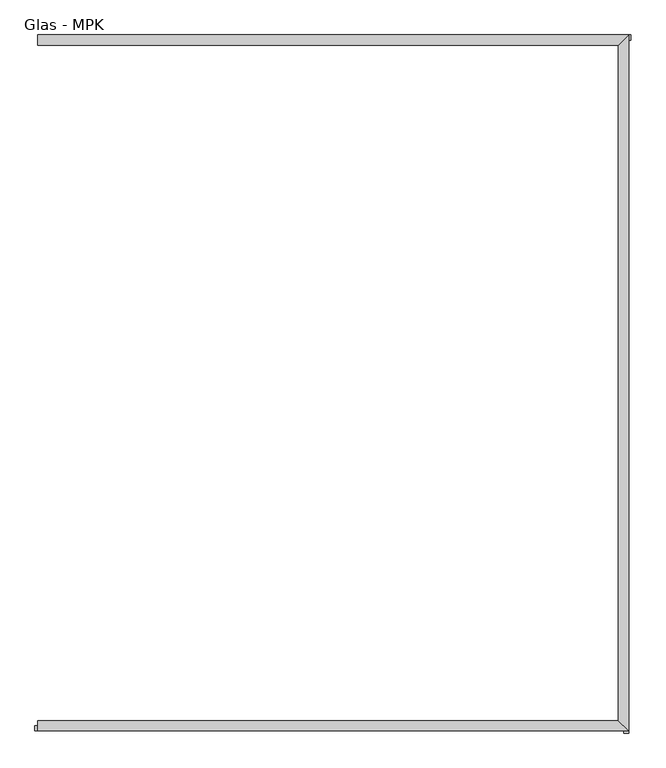
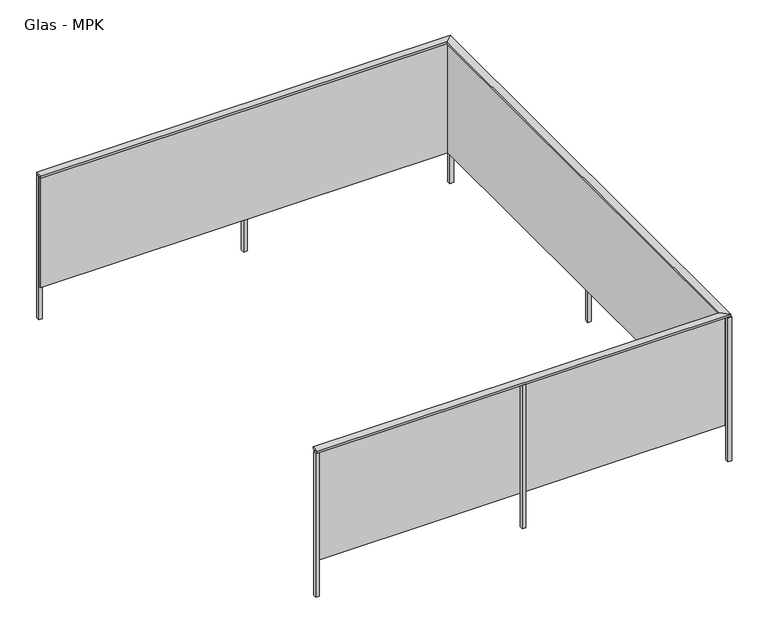
"""IFC4 building model written with IfcOpenShell, lengths in millimetres: railing geometry, Glas - MPK."""

import ifcopenshell
import ifcopenshell.guid

model = None  # the IFC model being written
_history = None  # IfcOwnerHistory: only IFC2X3 demands one
_inside = {}  # id of a spatial element -> (the spatial element, [elements in it])
_under = {}  # id of a project, library or spatial element -> (it, [spatial elements below it])
_declared = {}  # id of a project -> (the project, [libraries it declares])
_typed = {}  # id of a type object -> (the type object, [elements of that type])
_made_of = {}  # id of a material, layer set ... -> (it, [elements and type objects made of it])


def new_model(schema):
    """Start an empty IFC model of exactly this schema.

    Asked for "IFC4X3", IfcOpenShell would pick the latest addendum, in which some entities
    have other attributes; the version numbers below select the first issue.
    IFC2X3 requires an IfcOwnerHistory on every rooted entity: one is made here for all.
    """
    global model, _history
    if schema == "IFC4X3":
        model = ifcopenshell.file(schema_version=(4, 3, 0, 0))
    else:
        model = ifcopenshell.file(schema=schema)
    _inside.clear()
    _under.clear()
    _declared.clear()
    _typed.clear()
    _made_of.clear()
    _history = None
    if model.schema == "IFC2X3":
        org = make("IfcOrganization", Name="unknown")
        user = make(
            "IfcPersonAndOrganization",
            ThePerson=make("IfcPerson", FamilyName="unknown"),
            TheOrganization=org,
        )
        app = make(
            "IfcApplication",
            ApplicationDeveloper=org,
            Version="unknown",
            ApplicationFullName="unknown",
            ApplicationIdentifier="unknown",
        )
        _history = make(
            "IfcOwnerHistory",
            OwningUser=user,
            OwningApplication=app,
            ChangeAction="ADDED",
            CreationDate=0,
        )
    return model


def make(cls, **values):
    """One entity of the class cls with the attributes given. An attribute that is None is left unset."""
    return model.create_entity(
        cls, **{name: value for name, value in values.items() if value is not None}
    )


def rooted(cls, **values):
    """An entity with a GlobalId (a new one), such as an element, a storey or a relation."""
    return make(cls, GlobalId=ifcopenshell.guid.new(), OwnerHistory=_history, **values)


def si_unit(unit_type, name, prefix=None):
    """IfcSIUnit, for example si_unit("LENGTHUNIT", "METRE", prefix="MILLI")."""
    return make("IfcSIUnit", UnitType=unit_type, Prefix=prefix, Name=name)


def assignment(units):
    """IfcUnitAssignment: the units of a project."""
    return None if units is None else make("IfcUnitAssignment", Units=units)


def point(xyz):
    """IfcCartesianPoint."""
    return None if xyz is None else make("IfcCartesianPoint", Coordinates=xyz)


def direction(xyz):
    """IfcDirection."""
    return None if xyz is None else make("IfcDirection", DirectionRatios=xyz)


def frame(location, z_axis=None, x_axis=None):
    """IfcAxis2Placement3D, a coordinate frame: its origin and axes. An axis left out is left unset."""
    return make(
        "IfcAxis2Placement3D",
        Location=point(location),
        Axis=direction(z_axis),
        RefDirection=direction(x_axis),
    )


def origin():
    """The frame at (0, 0, 0) with its axes left unset."""
    return frame((0.0, 0.0, 0.0))


def place(relative_to, where):
    """IfcLocalPlacement: puts the frame where relative to a parent placement (None: the world)."""
    return make(
        "IfcLocalPlacement", PlacementRelTo=relative_to, RelativePlacement=where
    )


def context(
    kind, dimensions, precision=None, world=None, true_north=None, identifier=None
):
    """IfcGeometricRepresentationContext, for example the 3D "Model" context."""
    return make(
        "IfcGeometricRepresentationContext",
        ContextIdentifier=identifier,
        ContextType=kind,
        CoordinateSpaceDimension=dimensions,
        Precision=precision,
        WorldCoordinateSystem=world,
        TrueNorth=true_north,
    )


def project(units=None, contexts=None):
    """IfcProject with its units and contexts."""
    return rooted(
        "IfcProject",
        Name="project",
        RepresentationContexts=contexts,
        UnitsInContext=assignment(units),
    )


def spatial(cls, under=None, at=None, **own):
    """A site, building, storey or space (cls), placed at a placement, below another one or the project."""
    s = rooted(cls, ObjectPlacement=at, **own)
    if under is not None:
        _under.setdefault(under.id(), (under, []))[1].append(s)
    return s


def polyline(points):
    """IfcPolyline through the points."""
    return make("IfcPolyline", Points=[point(p) for p in points])


def outline(outer, holes=None, kind="AREA"):
    """IfcArbitraryClosedProfileDef: a profile drawn as a closed curve; with holes, ...WithVoids."""
    if holes is None:
        return make("IfcArbitraryClosedProfileDef", ProfileType=kind, OuterCurve=outer)
    return make(
        "IfcArbitraryProfileDefWithVoids",
        ProfileType=kind,
        OuterCurve=outer,
        InnerCurves=holes,
    )


def extrude(swept, where, along, depth):
    """IfcExtrudedAreaSolid: the profile swept, set in the frame where, extruded along a direction by depth."""
    return make(
        "IfcExtrudedAreaSolid",
        SweptArea=swept,
        Position=where,
        ExtrudedDirection=direction(along),
        Depth=depth,
    )


def faces_of(points, faces, orient=None, outer=None):
    """IfcFace entities. A face is a list of loops; a loop is a list of indices into points, from 0.

    orient and outer hold one flag for each loop. By default every Orientation is true, the
    first loop of a face is its IfcFaceOuterBound and the others are IfcFaceBound.
    """
    made = []
    for i, loops in enumerate(faces):
        bounds = []
        for j, loop in enumerate(loops):
            is_outer = j == 0 if outer is None else outer[i][j]
            bounds.append(
                make(
                    "IfcFaceOuterBound" if is_outer else "IfcFaceBound",
                    Bound=make("IfcPolyLoop", Polygon=[points[k] for k in loop]),
                    Orientation=True if orient is None else orient[i][j],
                )
            )
        made.append(make("IfcFace", Bounds=bounds))
    return made


def faceted_brep(points, faces, orient=None, outer=None, voids=None):
    """IfcFacetedBrep: a solid bounded by flat faces; with voids (closed shells), ...WithVoids."""
    shared = [point(p) for p in points]
    hull = make("IfcClosedShell", CfsFaces=faces_of(shared, faces, orient, outer))
    if voids is None:
        return make("IfcFacetedBrep", Outer=hull)
    return make(
        "IfcFacetedBrepWithVoids",
        Outer=hull,
        Voids=[
            make(cls, CfsFaces=faces_of(shared, fs, o, b)) for cls, fs, o, b in voids
        ],
    )


def shape(context_of_items, identifier, shape_type, items):
    """IfcShapeRepresentation: the items that make up one representation, for example the "Body"."""
    return make(
        "IfcShapeRepresentation",
        ContextOfItems=context_of_items,
        RepresentationIdentifier=identifier,
        RepresentationType=shape_type,
        Items=items,
    )


def source(mapping_origin, context_of_items, identifier, shape_type, items):
    """IfcRepresentationMap: a shape defined once, which mapped items show again and again."""
    return make(
        "IfcRepresentationMap",
        MappingOrigin=mapping_origin,
        MappedRepresentation=shape(context_of_items, identifier, shape_type, items),
    )


def transform(
    local_origin,
    x_axis=None,
    y_axis=None,
    z_axis=None,
    scale=None,
    scale2=None,
    scale3=None,
    uniform=True,
):
    """IfcCartesianTransformationOperator3D, or its non-uniform kind. x_axis, y_axis, z_axis: its Axis1, 2, 3."""
    if uniform:
        return make(
            "IfcCartesianTransformationOperator3D",
            Axis1=direction(x_axis),
            Axis2=direction(y_axis),
            LocalOrigin=point(local_origin),
            Scale=scale,
            Axis3=direction(z_axis),
        )
    return make(
        "IfcCartesianTransformationOperator3DnonUniform",
        Axis1=direction(x_axis),
        Axis2=direction(y_axis),
        LocalOrigin=point(local_origin),
        Scale=scale,
        Axis3=direction(z_axis),
        Scale2=scale2,
        Scale3=scale3,
    )


def mapped(mapping_source, mapping_target):
    """IfcMappedItem: shows the shape of a source again, moved by a transform."""
    return make(
        "IfcMappedItem", MappingSource=mapping_source, MappingTarget=mapping_target
    )


def made_of(thing, what):
    """Note that an element or type object is made of a material, layer set ...; save() writes the relation."""
    if what is not None:
        _made_of.setdefault(what.id(), (what, []))[1].append(thing)
    return thing


def element(
    cls,
    number,
    at=None,
    inside=None,
    cuts=None,
    type_object=None,
    material=None,
    context=None,
    identifier="Body",
    shape_type=None,
    held_by="IfcProductDefinitionShape",
    body=None,
    shapes=None,
    **own,
):
    """One element of the class cls, such as IfcWall. Its Tag is "e" and its number.

    at: its placement. inside: the storey or other place that contains it. cuts: it is an
    opening in that element (IfcRelVoidsElement). A single representation is given by context,
    identifier, shape_type and body (its items); several are given by shapes. held_by: the class
    of the entity that holds the representations. save() writes the other relations.
    """
    e = rooted(cls, Tag="e%d" % number, ObjectPlacement=at, **own)
    if body is not None:
        shapes = [shape(context, identifier, shape_type, body)]
    if shapes is not None:
        e.Representation = make(held_by, Representations=shapes)
    if inside is not None:
        _inside.setdefault(inside.id(), (inside, []))[1].append(e)
    if cuts is not None:
        rooted(
            "IfcRelVoidsElement", RelatingBuildingElement=cuts, RelatedOpeningElement=e
        )
    if type_object is not None:
        _typed.setdefault(type_object.id(), (type_object, []))[1].append(e)
    return made_of(e, material)


def aggregate(whole, parts):
    """IfcRelAggregates: a whole, such as a stair, and the parts it consists of."""
    return rooted("IfcRelAggregates", RelatingObject=whole, RelatedObjects=parts)


def save(model, path):
    """Write the relations noted so far, then the file.

    IfcRelAggregates (storeys below a building ...), IfcRelContainedInSpatialStructure (elements
    in a storey), IfcRelDefinesByType, IfcRelAssociatesMaterial and IfcRelDeclares: one each for
    every whole, place, type object, material and project.
    """
    for whole, parts in _under.values():
        aggregate(whole, parts)
    for where, things in _inside.values():
        rooted(
            "IfcRelContainedInSpatialStructure",
            RelatedElements=things,
            RelatingStructure=where,
        )
    for kind, things in _typed.values():
        rooted("IfcRelDefinesByType", RelatedObjects=things, RelatingType=kind)
    for what, things in _made_of.values():
        rooted("IfcRelAssociatesMaterial", RelatedObjects=things, RelatingMaterial=what)
    for by, libraries in _declared.values():
        rooted("IfcRelDeclares", RelatingContext=by, RelatedDefinitions=libraries)
    model.write(path)


def glas_mpk_ffa405cb(model_context):
    return source(origin(), model_context, "Body", "SolidModel", [
        faceted_brep([(29194.1667192, -1196.642277, 12843.2628643), (29194.1667192, -1246.642277, 12843.2628643), (29194.1667192, -1246.642277, 12856.7371357), (29194.1667192, -1196.642277, 12856.7371357), (32034.1667192, -1196.642277, 12843.2628643), (31984.1667192, -1246.642277, 12843.2628643), (31984.1667192, -1246.642277, 12856.7371357), (32034.1667192, -1196.642277, 12856.7371357), (32034.1667192, -4537.3716232, 12843.2628643), (31984.1667192, -4487.3716232, 12843.2628643), (31984.1667192, -4487.3716232, 12856.7371357), (32034.1667192, -4537.3716232, 12856.7371357), (29194.1667192, -4537.3716232, 12843.2628643), (29194.1667192, -4537.3716232, 12856.7371357), (29194.1667192, -4487.3716232, 12856.7371357), (29194.1667192, -4487.3716232, 12843.2628643)], [[[0, 1, 2, 3]], [[1, 0, 4, 5]], [[2, 1, 5, 6]], [[3, 2, 6, 7]], [[0, 3, 7, 4]], [[5, 4, 8, 9]], [[6, 5, 9, 10]], [[7, 6, 10, 11]], [[4, 7, 11, 8]], [[12, 13, 14, 15]], [[9, 8, 12, 15]], [[10, 9, 15, 14]], [[11, 10, 14, 13]], [[8, 11, 13, 12]]]),
        faceted_brep([(29194.1667192, -1236.642277, 12842.8769824), (29194.1667192, -1222.4501531, 12842.8769824), (29194.1667192, -1222.4501531, 12042.8769824), (29194.1667192, -1236.642277, 12042.8769824), (31994.1667192, -1236.642277, 12842.8769824), (32008.3588432, -1222.4501531, 12842.8769824), (32008.3588432, -1222.4501531, 12042.8769824), (31994.1667192, -1236.642277, 12042.8769824), (31994.1667192, -4497.3716232, 12842.8769824), (32008.3588432, -4511.5637472, 12842.8769824), (32008.3588432, -4511.5637472, 12042.8769824), (31994.1667192, -4497.3716232, 12042.8769824), (29194.1667192, -4497.3716232, 12842.8769824), (29194.1667192, -4497.3716232, 12042.8769824), (29194.1667192, -4511.5637472, 12042.8769824), (29194.1667192, -4511.5637472, 12842.8769824)], [[[0, 1, 2, 3]], [[1, 0, 4, 5]], [[2, 1, 5, 6]], [[3, 2, 6, 7]], [[0, 3, 7, 4]], [[5, 4, 8, 9]], [[6, 5, 9, 10]], [[7, 6, 10, 11]], [[4, 7, 11, 8]], [[12, 13, 14, 15]], [[9, 8, 12, 15]], [[10, 9, 15, 14]], [[11, 10, 14, 13]], [[8, 11, 13, 12]]]),
        extrude(outline(polyline([(30625.4167192, -4512.3716232), (30625.4167192, -4537.3716232), (30600.4167192, -4537.3716232), (30600.4167192, -4512.3716232), (30625.4167192, -4512.3716232)])), frame((0.0, 0.0, 11800.0), z_axis=(0.0, 0.0, 1.0), x_axis=(1.0, 0.0, 0.0)), (0.0, 0.0, 1.0), 1043.2628643),
        extrude(outline(polyline([(32009.1667192, -2854.5069501), (32034.1667192, -2854.5069501), (32034.1667192, -2879.5069501), (32009.1667192, -2879.5069501), (32009.1667192, -2854.5069501)])), frame((0.0, 0.0, 11800.0), z_axis=(0.0, 0.0, 1.0), x_axis=(1.0, 0.0, 0.0)), (0.0, 0.0, 1.0), 1043.2628643),
        extrude(outline(polyline([(30600.4167192, -1221.642277), (30600.4167192, -1196.642277), (30625.4167192, -1196.642277), (30625.4167192, -1221.642277), (30600.4167192, -1221.642277)])), frame((0.0, 0.0, 11800.0), z_axis=(0.0, 0.0, 1.0), x_axis=(1.0, 0.0, 0.0)), (0.0, 0.0, 1.0), 1043.2628643),
        extrude(outline(polyline([(32009.1667192, -4522.3716232), (32034.1667192, -4522.3716232), (32034.1667192, -4547.3716232), (32009.1667192, -4547.3716232), (32009.1667192, -4522.3716232)])), frame((0.0, 0.0, 11800.0), z_axis=(0.0, 0.0, 1.0), x_axis=(1.0, 0.0, 0.0)), (0.0, 0.0, 1.0), 1043.2628643),
        extrude(outline(polyline([(32019.1667192, -1221.642277), (32019.1667192, -1196.642277), (32044.1667192, -1196.642277), (32044.1667192, -1221.642277), (32019.1667192, -1221.642277)])), frame((0.0, 0.0, 11800.0), z_axis=(0.0, 0.0, 1.0), x_axis=(1.0, 0.0, 0.0)), (0.0, 0.0, 1.0), 1043.2628643),
        extrude(outline(polyline([(29206.6667192, -4512.3716232), (29206.6667192, -4537.3716232), (29181.6667192, -4537.3716232), (29181.6667192, -4512.3716232), (29206.6667192, -4512.3716232)])), frame((0.0, 0.0, 11800.0), z_axis=(0.0, 0.0, 1.0), x_axis=(1.0, 0.0, 0.0)), (0.0, 0.0, 1.0), 1043.2628643),
        extrude(outline(polyline([(29194.1667192, -1221.642277), (29194.1667192, -1196.642277), (29219.1667192, -1196.642277), (29219.1667192, -1221.642277), (29194.1667192, -1221.642277)])), frame((0.0, 0.0, 11800.0), z_axis=(0.0, 0.0, 1.0), x_axis=(1.0, 0.0, 0.0)), (0.0, 0.0, 1.0), 1043.2628643),
    ])


if __name__ == "__main__":
    model = new_model("IFC4")
    model_context = context("Model", 3, world=origin())
    ifc_project = project(units=[si_unit("LENGTHUNIT", "METRE", prefix="MILLI")], contexts=[model_context])
    site = spatial("IfcSite", under=ifc_project)
    building = spatial("IfcBuilding", under=site)
    placement = place(None, origin())
    glas_mpk_shape = glas_mpk_ffa405cb(model_context)
    element("IfcRailing", 1, ObjectType="Glas - MPK", at=placement, inside=building, context=model_context, shape_type="MappedRepresentation", body=[
        mapped(glas_mpk_shape, transform((0.0, 0.0, 0.0), x_axis=(1.0, 0.0, 0.0), y_axis=(0.0, 1.0, 0.0), z_axis=(0.0, 0.0, 1.0))),
    ])
    save(model, "model.ifc")

# Revit data of these elements
# Element 1 (IfcRailing, "Glas - MPK")
#   Materials on its faces: "Metal - Aluminum", "Window - Glass"
# Materials
#   "Metal - Aluminum": class "Unassigned", colour RGB 247 247 247, transparency 0, Comments = "Rendering appearance not upgraded "
#   "Window - Glass": class "Glas", colour RGB 128 128 255, transparency 0.75
